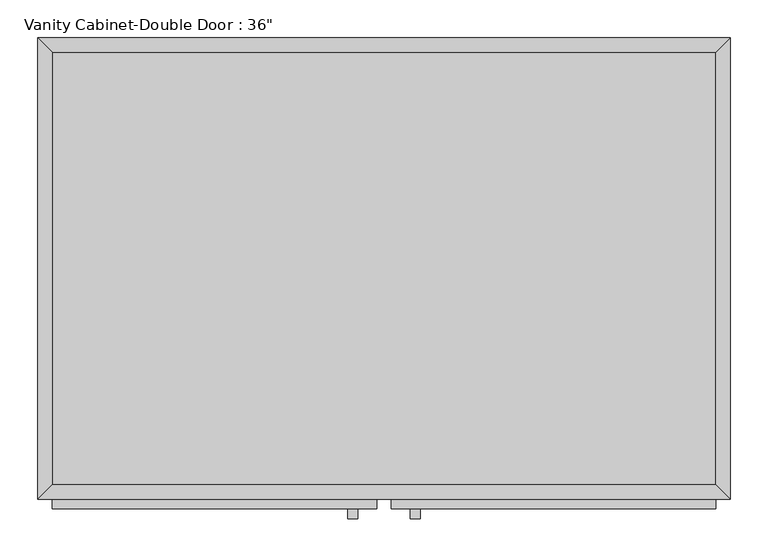
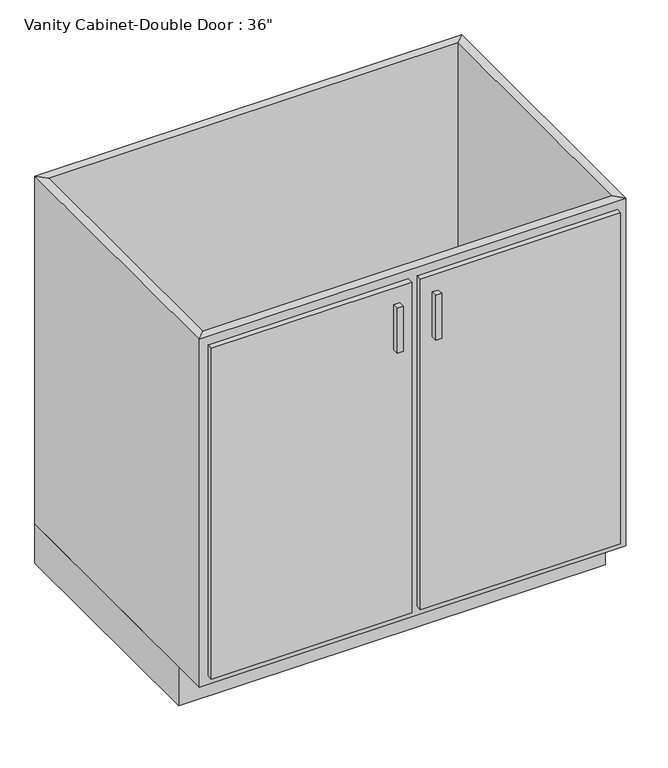
"""IFC4 building model written with IfcOpenShell, lengths in millimetres: furniture geometry."""

from ifc_helpers import new_model, si_unit, frame, origin, origin_with_axes, place, context, project, spatial, polyline, outline, extrude, faceted_brep, source, transform, mapped, element, save


def furniture_aeada037(model_context):
    return source(origin(), model_context, "Body", "SolidModel", [
        extrude(outline(polyline([(456.8877049, -19.05), (456.8877049, -590.55), (-419.4122951, -590.55), (-419.4122951, -19.05), (456.8877049, -19.05)])), frame((0.0, 0.0, 88.9), z_axis=(0.0, 0.0, 1.0), x_axis=(1.0, 0.0, 0.0)), (0.0, 0.0, 1.0), 19.05),
        faceted_brep([(456.8877049, -590.55, 876.3), (456.8877049, -590.55, 88.9), (-419.4122951, -590.55, 88.9), (-419.4122951, -590.55, 876.3), (475.9377049, -609.6, 876.3), (-438.4622951, -609.6, 876.3), (475.9377049, -609.6, 88.9), (-438.4622951, -609.6, 88.9), (-419.4122951, -19.05, 88.9), (-419.4122951, -19.05, 876.3), (-438.4622951, 0.0, 876.3), (-438.4622951, 0.0, 88.9), (456.8877049, -19.05, 88.9), (456.8877049, -19.05, 876.3), (475.9377049, 0.0, 876.3), (475.9377049, 0.0, 88.9)], [[[0, 1, 2, 3]], [[4, 0, 3, 5]], [[6, 4, 5, 7]], [[1, 6, 7, 2]], [[3, 2, 8, 9]], [[5, 3, 9, 10]], [[7, 5, 10, 11]], [[2, 7, 11, 8]], [[9, 8, 12, 13]], [[10, 9, 13, 14]], [[11, 10, 14, 15]], [[8, 11, 15, 12]], [[13, 12, 1, 0]], [[14, 13, 0, 4]], [[15, 14, 4, 6]], [[12, 15, 6, 1]]]),
        extrude(outline(polyline([(475.9377049, 0.0), (475.9377049, -533.4), (-438.4622951, -533.4), (-438.4622951, 0.0), (475.9377049, 0.0)])), origin_with_axes(), (0.0, 0.0, 1.0), 88.9),
        extrude(outline(polyline([(-16.1872951, -635.0), (-28.8872951, -635.0), (-28.8872951, -622.3), (-16.1872951, -622.3), (-16.1872951, -635.0)])), frame((0.0, 0.0, 717.55), z_axis=(0.0, 0.0, 1.0), x_axis=(1.0, 0.0, 0.0)), (0.0, 0.0, 1.0), 101.6),
        extrude(outline(polyline([(66.3627049, -635.0), (53.6627049, -635.0), (53.6627049, -622.3), (66.3627049, -622.3), (66.3627049, -635.0)])), frame((0.0, 0.0, 717.55), z_axis=(0.0, 0.0, 1.0), x_axis=(1.0, 0.0, 0.0)), (0.0, 0.0, 1.0), 101.6),
        extrude(outline(polyline([(9.2127049, -622.3), (-419.4122951, -622.3), (-419.4122951, -609.6), (9.2127049, -609.6), (9.2127049, -622.3)])), frame((0.0, 0.0, 107.95), z_axis=(0.0, 0.0, 1.0), x_axis=(1.0, 0.0, 0.0)), (0.0, 0.0, 1.0), 749.3),
        extrude(outline(polyline([(456.8877049, -622.3), (28.2627049, -622.3), (28.2627049, -609.6), (456.8877049, -609.6), (456.8877049, -622.3)])), frame((0.0, 0.0, 107.95), z_axis=(0.0, 0.0, 1.0), x_axis=(1.0, 0.0, 0.0)), (0.0, 0.0, 1.0), 749.3),
    ])


if __name__ == "__main__":
    model = new_model("IFC4")
    model_context = context("Model", 3, world=origin())
    ifc_project = project(units=[si_unit("LENGTHUNIT", "METRE", prefix="MILLI")], contexts=[model_context])
    site = spatial("IfcSite", under=ifc_project)
    building = spatial("IfcBuilding", under=site)
    placement = place(None, origin())
    furniture_shape = furniture_aeada037(model_context)
    element("IfcFurniture", 1, ObjectType="Vanity Cabinet-Double Door : 36\"", at=placement, inside=building, context=model_context, shape_type="MappedRepresentation", body=[
        mapped(furniture_shape, transform((0.0, 0.0, 0.0), x_axis=(1.0, 0.0, 0.0), y_axis=(0.0, 1.0, 0.0), z_axis=(0.0, 0.0, 1.0))),
    ])
    save(model, "model.ifc")

# Revit data of these elements
# Type "Vanity Cabinet-Double Door : 36\""
#   Finish = "Cabinetry"
#   Assembly Code = "C1030410"
#   Depth = 2' - 0"
#   Height = 2' - 10 1/2"
#   Toe Depth = 0' - 3"
#   Toe Height = 0' - 3 1/2"
#   Width = 3' - 0"
#   Cabinet Material = Cabinets
#   Door/Drawer Material = Cabinets
#   Handle Material = Cabinets - Handles
# Element 1 (IfcFurniture, "Vanity Cabinet-Double Door : 36\"")
#   Materials on its faces: "Cabinets", "Cabinets - Handles"
# Materials
#   "Cabinets": class "Paint", colour RGB 249 249 249, transparency 0
#   "Cabinets - Handles": class "Metal", colour RGB 57 57 57, transparency 0
